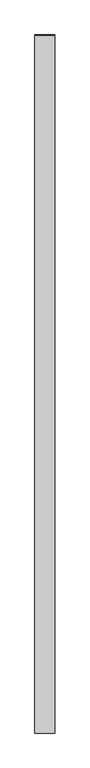
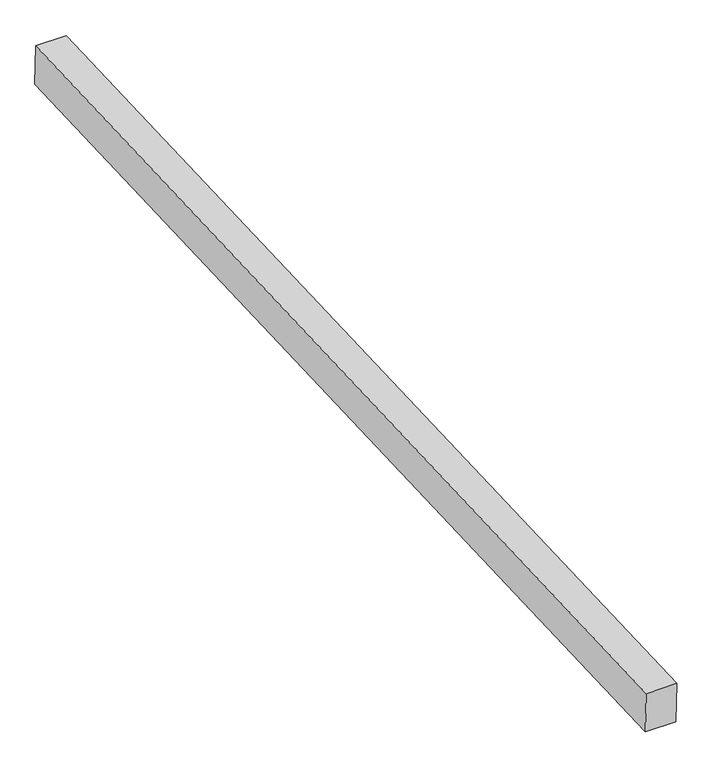
"""IFC4 building model written with IfcOpenShell, lengths in millimetres: proxy geometry, Generic Models 7:Generic Models 1:8:Generic Models 1:8 : Generic Models 7:Generic Models 1:337419:48 : Generic Models 7:Generic Models 1:8:Generic Models 1:8 : Generic Models 7:Generic Models 1:337419:315935."""

from ifc_helpers import new_model, si_unit, frame, origin, place, context, project, spatial, polyline, outline, extrude, source, transform, mapped, element, save


def generic_models_f6bb88ea(model_context):
    return source(origin(), model_context, "Body", "SweptSolid", [
        extrude(outline(polyline([(-581229.2495411, 3818.908703), (-576356.3266468, 4021.9471569), (-576348.7597251, 3831.5971524), (-581221.3189223, 3628.5738526), (-581229.2495411, 3818.908703)])), frame((612048.311724, 0.0, 0.0), z_axis=(1.0, 0.0, 0.0), x_axis=(0.0, 1.0, 0.0)), (0.0, 0.0, 1.0), 139.7),
    ])


if __name__ == "__main__":
    model = new_model("IFC4")
    model_context = context("Model", 3, world=origin())
    ifc_project = project(units=[si_unit("LENGTHUNIT", "METRE", prefix="MILLI")], contexts=[model_context])
    site = spatial("IfcSite", under=ifc_project)
    building = spatial("IfcBuilding", under=site)
    placement = place(None, origin())
    generic_models_shape = generic_models_f6bb88ea(model_context)
    element("IfcBuildingElementProxy", 1, Name="Generic Models 7:Generic Models 1:8:Generic Models 1:8 : Generic Models 7:Generic Models 1:337419:48 : Generic Models 7:Generic Models 1:8:Generic Models 1:8 : Generic Models 7:Generic Models 1:337419:315935", ObjectType="Generic Models 7:Generic Models 1:8:Generic Models 1:8 : Generic Models 7:Generic Models 1:337419:48 : Generic Models 7:Generic Models 1:8:Generic Models 1:8 : Generic Models 7:Generic Models 1:337419:315935", at=placement, inside=building, context=model_context, shape_type="MappedRepresentation", body=[
        mapped(generic_models_shape, transform((0.0, 0.0, 0.0), x_axis=(1.0, 0.0, 0.0), y_axis=(0.0, 1.0, 0.0), z_axis=(0.0, 0.0, 1.0))),
    ])
    save(model, "model.ifc")

# Revit data of these elements
# Type "Generic Models 7:Generic Models 1:8:Generic Models 1:8 : Generic Models 7:Generic Models 1:337419:48 : Generic Models 7:Generic Models 1:8:Generic Models 1:8 : Generic Models 7:Generic Models 1:337419:315935"
#   NameOverride = "Generic Models 7:Generic Models 1:8:Generic Models 1:8 : Generic Models 7:Generic Models 1:337419:315935"
#   ObjectTypeOverride = "Generic Models 1:8 : Generic Models 7:Generic Models 1:337419"
#   Reference = "Generic Models 1"
#   Tag = "315935"
# Element 1 (IfcBuildingElementProxy, "Generic Models 7:Generic Models 1:8:Generic Models 1:8 : Generic Models 7:Generic Models 1:337419:48 : Generic Models 7:Generic Models 1:8:Generic Models 1:8 : Generic Models 7:Generic Models 1:337419:315935")
#   Materials on its faces: "5 1/2\" X 7 1/2\" EXTERIOR GRADE GLULAM BEAMS"
# Materials
#   "5 1/2\" X 7 1/2\" EXTERIOR GRADE GLULAM BEAMS": class "Wood", colour RGB 183 134 68, transparency 0, Keynote = "M06181300.01", Description = "Pinus Echinata", Cost = 0
